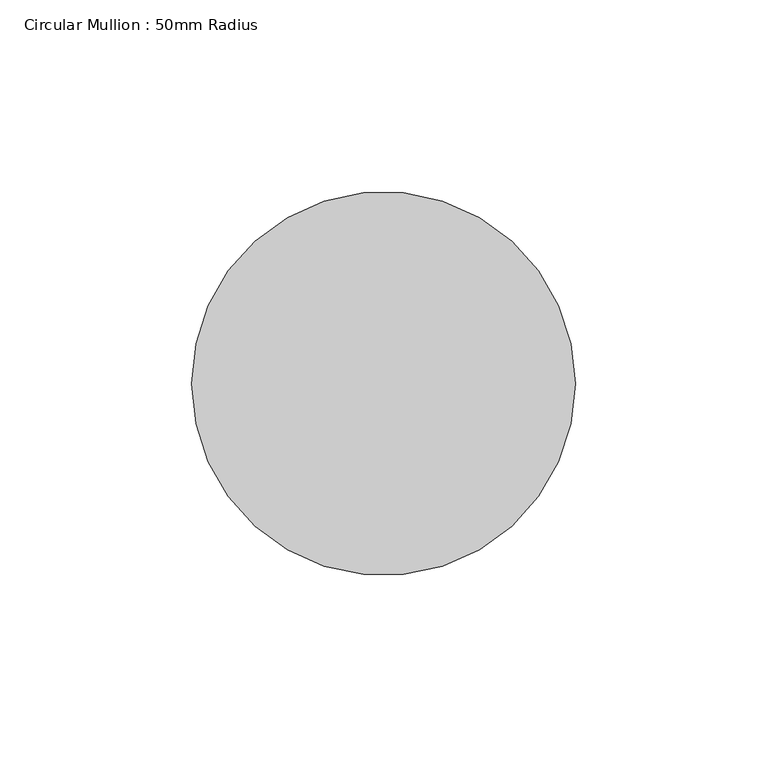
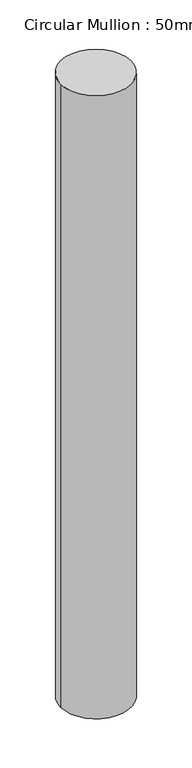
"""IFC4 building model written with IfcOpenShell, lengths in millimetres: member geometry, Circular Mullion : 50mm Radius."""

from ifc_helpers import new_model, si_unit, point, frame, origin, origin_2d, place, context, project, spatial, circle_curve, trimmed, segment, composite_curve, outline, extrude, source, transform, mapped, element, save


def circular_mullion_50mm_radius_7a4ad373(model_context):
    return source(origin(), model_context, "Body", "SweptSolid", [
        extrude(outline(composite_curve([segment(trimmed(circle_curve(origin_2d(), 50.0), [point((50.0, 0.0))], [point((-50.0, 0.0))], False, "CARTESIAN"), True, "CONTINUOUS"), segment(trimmed(circle_curve(origin_2d(), 50.0), [point((-50.0, 0.0))], [point((50.0, 0.0))], False, "CARTESIAN"), True, "CONTINUOUS")], self_intersect=False)), frame((0.0, 0.0, -936.5687182), z_axis=(0.0, 0.0, 1.0), x_axis=(1.0, 0.0, 0.0)), (0.0, 0.0, 1.0), 936.5687182),
    ])


if __name__ == "__main__":
    model = new_model("IFC4")
    model_context = context("Model", 3, world=origin())
    ifc_project = project(units=[si_unit("LENGTHUNIT", "METRE", prefix="MILLI")], contexts=[model_context])
    site = spatial("IfcSite", under=ifc_project)
    building = spatial("IfcBuilding", under=site)
    placement = place(None, origin())
    circular_mullion_50mm_radius_shape = circular_mullion_50mm_radius_7a4ad373(model_context)
    element("IfcMember", 1, ObjectType="Circular Mullion : 50mm Radius", at=placement, inside=building, context=model_context, shape_type="MappedRepresentation", body=[
        mapped(circular_mullion_50mm_radius_shape, transform((0.0, 0.0, 0.0), x_axis=(1.0, 0.0, 0.0), y_axis=(0.0, 1.0, 0.0), z_axis=(0.0, 0.0, 1.0))),
    ])
    save(model, "model.ifc")

# Revit data of these elements
# Type "Circular Mullion : 50mm Radius"
#   built-in parameter 1007350 = 0.164042 (stored number, unit not read)
# Element 1 (IfcMember, "Circular Mullion : 50mm Radius")
#   Materials on its faces: "Aluminium"
# Materials
#   "Aluminium": class "Metal", colour RGB 247 247 247, transparency 0, Description = "Aluminium 6061", Cost = 0
